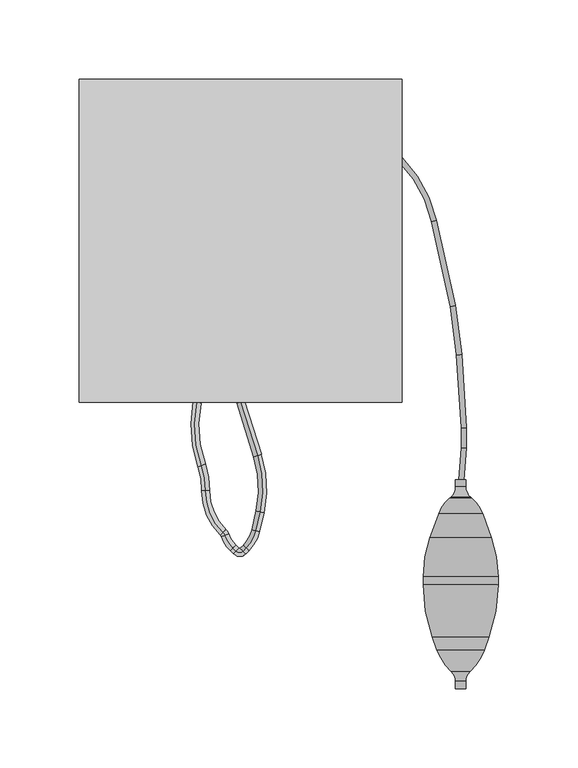
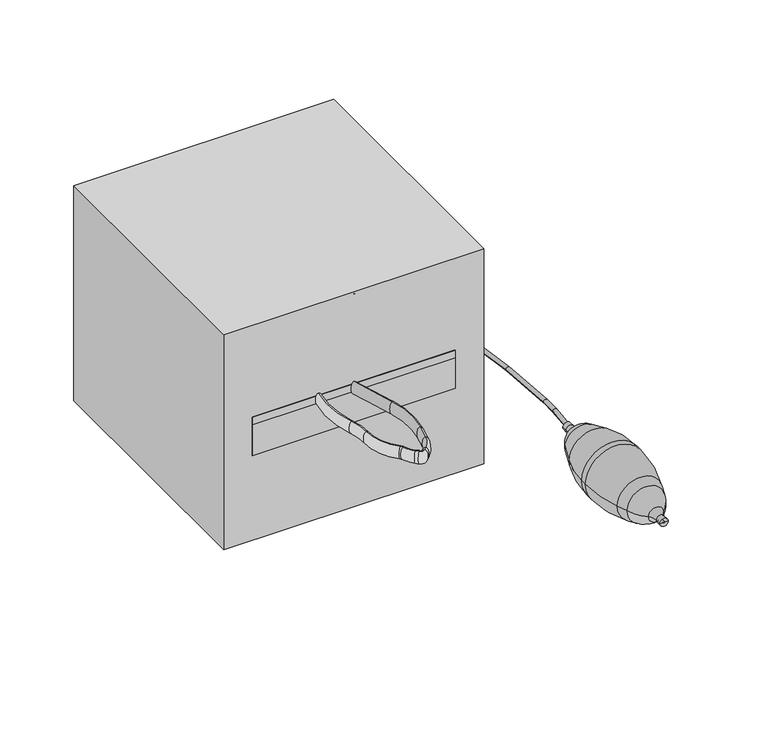
"""IFC4 building model written with IfcOpenShell, lengths in millimetres: proxy geometry, M4100 - Sphygmomanometer, Aneroid, Wall-Mounted : M4100 - Sphygmomanometer, Aneroid, Wall-Mounted."""

import ifcopenshell
import ifcopenshell.guid

model = None  # the IFC model being written
_history = None  # IfcOwnerHistory: only IFC2X3 demands one
_inside = {}  # id of a spatial element -> (the spatial element, [elements in it])
_under = {}  # id of a project, library or spatial element -> (it, [spatial elements below it])
_declared = {}  # id of a project -> (the project, [libraries it declares])
_typed = {}  # id of a type object -> (the type object, [elements of that type])
_made_of = {}  # id of a material, layer set ... -> (it, [elements and type objects made of it])


def new_model(schema):
    """Start an empty IFC model of exactly this schema.

    Asked for "IFC4X3", IfcOpenShell would pick the latest addendum, in which some entities
    have other attributes; the version numbers below select the first issue.
    IFC2X3 requires an IfcOwnerHistory on every rooted entity: one is made here for all.
    """
    global model, _history
    if schema == "IFC4X3":
        model = ifcopenshell.file(schema_version=(4, 3, 0, 0))
    else:
        model = ifcopenshell.file(schema=schema)
    _inside.clear()
    _under.clear()
    _declared.clear()
    _typed.clear()
    _made_of.clear()
    _history = None
    if model.schema == "IFC2X3":
        org = make("IfcOrganization", Name="unknown")
        user = make(
            "IfcPersonAndOrganization",
            ThePerson=make("IfcPerson", FamilyName="unknown"),
            TheOrganization=org,
        )
        app = make(
            "IfcApplication",
            ApplicationDeveloper=org,
            Version="unknown",
            ApplicationFullName="unknown",
            ApplicationIdentifier="unknown",
        )
        _history = make(
            "IfcOwnerHistory",
            OwningUser=user,
            OwningApplication=app,
            ChangeAction="ADDED",
            CreationDate=0,
        )
    return model


def make(cls, **values):
    """One entity of the class cls with the attributes given. An attribute that is None is left unset."""
    return model.create_entity(
        cls, **{name: value for name, value in values.items() if value is not None}
    )


def rooted(cls, **values):
    """An entity with a GlobalId (a new one), such as an element, a storey or a relation."""
    return make(cls, GlobalId=ifcopenshell.guid.new(), OwnerHistory=_history, **values)


def si_unit(unit_type, name, prefix=None):
    """IfcSIUnit, for example si_unit("LENGTHUNIT", "METRE", prefix="MILLI")."""
    return make("IfcSIUnit", UnitType=unit_type, Prefix=prefix, Name=name)


def assignment(units):
    """IfcUnitAssignment: the units of a project."""
    return None if units is None else make("IfcUnitAssignment", Units=units)


def point(xyz):
    """IfcCartesianPoint."""
    return None if xyz is None else make("IfcCartesianPoint", Coordinates=xyz)


def direction(xyz):
    """IfcDirection."""
    return None if xyz is None else make("IfcDirection", DirectionRatios=xyz)


def frame(location, z_axis=None, x_axis=None):
    """IfcAxis2Placement3D, a coordinate frame: its origin and axes. An axis left out is left unset."""
    return make(
        "IfcAxis2Placement3D",
        Location=point(location),
        Axis=direction(z_axis),
        RefDirection=direction(x_axis),
    )


def frame_2d(location, x_axis=None):
    """IfcAxis2Placement2D, a coordinate frame in the plane: its origin and x axis."""
    return make(
        "IfcAxis2Placement2D", Location=point(location), RefDirection=direction(x_axis)
    )


def origin():
    """The frame at (0, 0, 0) with its axes left unset."""
    return frame((0.0, 0.0, 0.0))


def origin_with_axes():
    """The frame at (0, 0, 0) with the z axis (0, 0, 1) and the x axis (1, 0, 0) written out."""
    return frame((0.0, 0.0, 0.0), z_axis=(0.0, 0.0, 1.0), x_axis=(1.0, 0.0, 0.0))


def place(relative_to, where):
    """IfcLocalPlacement: puts the frame where relative to a parent placement (None: the world)."""
    return make(
        "IfcLocalPlacement", PlacementRelTo=relative_to, RelativePlacement=where
    )


def context(
    kind, dimensions, precision=None, world=None, true_north=None, identifier=None
):
    """IfcGeometricRepresentationContext, for example the 3D "Model" context."""
    return make(
        "IfcGeometricRepresentationContext",
        ContextIdentifier=identifier,
        ContextType=kind,
        CoordinateSpaceDimension=dimensions,
        Precision=precision,
        WorldCoordinateSystem=world,
        TrueNorth=true_north,
    )


def project(units=None, contexts=None):
    """IfcProject with its units and contexts."""
    return rooted(
        "IfcProject",
        Name="project",
        RepresentationContexts=contexts,
        UnitsInContext=assignment(units),
    )


def spatial(cls, under=None, at=None, **own):
    """A site, building, storey or space (cls), placed at a placement, below another one or the project."""
    s = rooted(cls, ObjectPlacement=at, **own)
    if under is not None:
        _under.setdefault(under.id(), (under, []))[1].append(s)
    return s


def polyline(points):
    """IfcPolyline through the points."""
    return make("IfcPolyline", Points=[point(p) for p in points])


def circle_curve(where, radius):
    """IfcCircle in the frame where."""
    return make("IfcCircle", Position=where, Radius=radius)


def ellipse_curve(where, semi_axis1, semi_axis2):
    """IfcEllipse in the frame where."""
    return make(
        "IfcEllipse", Position=where, SemiAxis1=semi_axis1, SemiAxis2=semi_axis2
    )


def trimmed(basis, trim1, trim2, sense, master):
    """IfcTrimmedCurve: the piece of a basis curve between two trims."""
    return make(
        "IfcTrimmedCurve",
        BasisCurve=basis,
        Trim1=trim1,
        Trim2=trim2,
        SenseAgreement=sense,
        MasterRepresentation=master,
    )


def segment(curve, same_sense, transition):
    """IfcCompositeCurveSegment."""
    return make(
        "IfcCompositeCurveSegment",
        Transition=transition,
        SameSense=same_sense,
        ParentCurve=curve,
    )


def composite_curve(segments, self_intersect=None):
    """IfcCompositeCurve: segments joined end to end."""
    return make("IfcCompositeCurve", Segments=segments, SelfIntersect=self_intersect)


def outline(outer, holes=None, kind="AREA"):
    """IfcArbitraryClosedProfileDef: a profile drawn as a closed curve; with holes, ...WithVoids."""
    if holes is None:
        return make("IfcArbitraryClosedProfileDef", ProfileType=kind, OuterCurve=outer)
    return make(
        "IfcArbitraryProfileDefWithVoids",
        ProfileType=kind,
        OuterCurve=outer,
        InnerCurves=holes,
    )


def extrude(swept, where, along, depth):
    """IfcExtrudedAreaSolid: the profile swept, set in the frame where, extruded along a direction by depth."""
    return make(
        "IfcExtrudedAreaSolid",
        SweptArea=swept,
        Position=where,
        ExtrudedDirection=direction(along),
        Depth=depth,
    )


def shape(context_of_items, identifier, shape_type, items):
    """IfcShapeRepresentation: the items that make up one representation, for example the "Body"."""
    return make(
        "IfcShapeRepresentation",
        ContextOfItems=context_of_items,
        RepresentationIdentifier=identifier,
        RepresentationType=shape_type,
        Items=items,
    )


def source(mapping_origin, context_of_items, identifier, shape_type, items):
    """IfcRepresentationMap: a shape defined once, which mapped items show again and again."""
    return make(
        "IfcRepresentationMap",
        MappingOrigin=mapping_origin,
        MappedRepresentation=shape(context_of_items, identifier, shape_type, items),
    )


def transform(
    local_origin,
    x_axis=None,
    y_axis=None,
    z_axis=None,
    scale=None,
    scale2=None,
    scale3=None,
    uniform=True,
):
    """IfcCartesianTransformationOperator3D, or its non-uniform kind. x_axis, y_axis, z_axis: its Axis1, 2, 3."""
    if uniform:
        return make(
            "IfcCartesianTransformationOperator3D",
            Axis1=direction(x_axis),
            Axis2=direction(y_axis),
            LocalOrigin=point(local_origin),
            Scale=scale,
            Axis3=direction(z_axis),
        )
    return make(
        "IfcCartesianTransformationOperator3DnonUniform",
        Axis1=direction(x_axis),
        Axis2=direction(y_axis),
        LocalOrigin=point(local_origin),
        Scale=scale,
        Axis3=direction(z_axis),
        Scale2=scale2,
        Scale3=scale3,
    )


def mapped(mapping_source, mapping_target):
    """IfcMappedItem: shows the shape of a source again, moved by a transform."""
    return make(
        "IfcMappedItem", MappingSource=mapping_source, MappingTarget=mapping_target
    )


def made_of(thing, what):
    """Note that an element or type object is made of a material, layer set ...; save() writes the relation."""
    if what is not None:
        _made_of.setdefault(what.id(), (what, []))[1].append(thing)
    return thing


def element(
    cls,
    number,
    at=None,
    inside=None,
    cuts=None,
    type_object=None,
    material=None,
    context=None,
    identifier="Body",
    shape_type=None,
    held_by="IfcProductDefinitionShape",
    body=None,
    shapes=None,
    **own,
):
    """One element of the class cls, such as IfcWall. Its Tag is "e" and its number.

    at: its placement. inside: the storey or other place that contains it. cuts: it is an
    opening in that element (IfcRelVoidsElement). A single representation is given by context,
    identifier, shape_type and body (its items); several are given by shapes. held_by: the class
    of the entity that holds the representations. save() writes the other relations.
    """
    e = rooted(cls, Tag="e%d" % number, ObjectPlacement=at, **own)
    if body is not None:
        shapes = [shape(context, identifier, shape_type, body)]
    if shapes is not None:
        e.Representation = make(held_by, Representations=shapes)
    if inside is not None:
        _inside.setdefault(inside.id(), (inside, []))[1].append(e)
    if cuts is not None:
        rooted(
            "IfcRelVoidsElement", RelatingBuildingElement=cuts, RelatedOpeningElement=e
        )
    if type_object is not None:
        _typed.setdefault(type_object.id(), (type_object, []))[1].append(e)
    return made_of(e, material)


def aggregate(whole, parts):
    """IfcRelAggregates: a whole, such as a stair, and the parts it consists of."""
    return rooted("IfcRelAggregates", RelatingObject=whole, RelatedObjects=parts)


def save(model, path):
    """Write the relations noted so far, then the file.

    IfcRelAggregates (storeys below a building ...), IfcRelContainedInSpatialStructure (elements
    in a storey), IfcRelDefinesByType, IfcRelAssociatesMaterial and IfcRelDeclares: one each for
    every whole, place, type object, material and project.
    """
    for whole, parts in _under.values():
        aggregate(whole, parts)
    for where, things in _inside.values():
        rooted(
            "IfcRelContainedInSpatialStructure",
            RelatedElements=things,
            RelatingStructure=where,
        )
    for kind, things in _typed.values():
        rooted("IfcRelDefinesByType", RelatedObjects=things, RelatingType=kind)
    for what, things in _made_of.values():
        rooted("IfcRelAssociatesMaterial", RelatedObjects=things, RelatingMaterial=what)
    for by, libraries in _declared.values():
        rooted("IfcRelDeclares", RelatingContext=by, RelatedDefinitions=libraries)
    model.write(path)


def plane_surface(at):
    """IfcPlane: the flat surface through the origin of the frame at, square to its z axis."""
    return make("IfcPlane", Position=at)


def cylinder_surface(at, radius):
    """IfcCylindricalSurface: all points at the distance radius from the z axis of the frame at."""
    return make("IfcCylindricalSurface", Position=at, Radius=radius)


def revolved_surface(curve, axis_point, axis_direction):
    """IfcSurfaceOfRevolution: the curve turned about the line through axis_point along axis_direction."""
    return make(
        "IfcSurfaceOfRevolution",
        SweptCurve=make("IfcArbitraryOpenProfileDef", ProfileType="CURVE", Curve=curve),
        AxisPosition=make("IfcAxis1Placement", Location=point(axis_point), Axis=direction(axis_direction)),
    )


def extruded_surface(curve, direction_of_extrusion, depth):
    """IfcSurfaceOfLinearExtrusion: the curve pushed along a direction by depth."""
    return make(
        "IfcSurfaceOfLinearExtrusion",
        SweptCurve=make("IfcArbitraryOpenProfileDef", ProfileType="CURVE", Curve=curve),
        ExtrudedDirection=direction(direction_of_extrusion),
        Depth=depth,
    )


def advanced_brep(points, edges, surfaces, faces):
    """IfcAdvancedBrep: a solid bounded by faces that lie on surfaces and meet in shared edges.

    An edge is (start, end): straight between two places in points (the first is 0);
    or (start, end, curve); or (start, end, curve, False) where it runs against its curve.
    A face is (place in surfaces, loops), or (place, loops, False) where it looks against
    its surface's normal. A loop lists edges by number (the first is 1), with a minus sign
    where the edge is run from its end to its start. The first loop is the outer one.
    """
    corners = [point(p) for p in points]
    vertices = [make("IfcVertexPoint", VertexGeometry=c) for c in corners]
    made = []
    for start, end, *more in edges:
        made.append(
            make(
                "IfcEdgeCurve",
                EdgeStart=vertices[start],
                EdgeEnd=vertices[end],
                EdgeGeometry=more[0] if more else make("IfcPolyline", Points=[corners[start], corners[end]]),
                SameSense=more[1] if len(more) > 1 else True,
            )
        )
    hull = []
    for where, loops, *sense in faces:
        bounds = []
        for j, loop in enumerate(loops):
            ring = [make("IfcOrientedEdge", EdgeElement=made[abs(k) - 1], Orientation=k > 0) for k in loop]
            bounds.append(
                make(
                    "IfcFaceOuterBound" if j == 0 else "IfcFaceBound",
                    Bound=make("IfcEdgeLoop", EdgeList=ring),
                    Orientation=True,
                )
            )
        hull.append(make("IfcAdvancedFace", Bounds=bounds, FaceSurface=surfaces[where], SameSense=sense[0] if sense else True))
    return make("IfcAdvancedBrep", Outer=make("IfcClosedShell", CfsFaces=hull))


def specialty_equipment_8f949246(model_context):
    return source(origin(), model_context, "Body", "SolidModel", [
        advanced_brep(
        [(0.0, 0.0, 93.3890108), (0.0, 0.0, 103.4609892), (10.60129, -33.4899695, 93.3890108), (10.60129, -33.4899695, 103.4609892), (12.1452256, -68.8519095, 103.4609892), (12.1452256, -68.8519095, 93.3890108), (9.4902706, -80.7634297, 93.3890108), (9.4902706, -80.7634297, 103.4609892), (3.5257448, -91.6206606, 103.4609892), (3.5257448, -91.6206606, 93.3890108), (1.489236, -93.6571694, 93.3890108), (1.489236, -93.6571694, 103.4609892), (-2.7411458, -93.6571694, 103.4609892), (-2.7411458, -93.6571694, 93.3890108), (-4.6658712, -91.732444, 93.3890108), (-4.6658712, -91.732444, 103.4609892), (-9.7582734, -83.8141156, 103.4609892), (-9.7582734, -83.8141156, 93.3890108), (-10.9708227, -81.9675873, 103.4609892), (-10.9708227, -81.9675873, 93.3890108), (-21.9594666, -55.7504476, 103.4609892), (-21.9594666, -55.7504476, 93.3890108), (-24.5939327, -39.9510684, 103.4609892), (-24.5939327, -39.9510684, 93.3890108), (-27.3580457, -0.1117834, 93.3890108), (-27.3580457, -0.1117834, 103.4609892)],
        [
            (0, 1, ellipse_curve(frame((0.0, 0.0, 98.425), z_axis=(-0.30179165133573443, 0.9533739031377199, 0.0), x_axis=(0.0, 0.0, 1.0)), 5.0359892, 2.5179946)),
            (1, 0, ellipse_curve(frame((0.0, 0.0, 98.425), z_axis=(-0.30179165133573443, 0.9533739031377199, 0.0), x_axis=(0.0, 0.0, 1.0)), 5.0359892, 2.5179946)),
            (0, 2),
            (2, 3, ellipse_curve(frame((10.60129, -33.4899695, 98.425), z_axis=(-0.3017916513357344, 0.9533739031377201, 0.0), x_axis=(0.0, 0.0, 1.0)), 5.0359892, 2.5179946)),
            (3, 1),
            (3, 2, ellipse_curve(frame((10.60129, -33.4899695, 98.425), z_axis=(-0.3017916513357344, 0.9533739031377201, 0.0), x_axis=(0.0, 0.0, 1.0)), 5.0359892, 2.5179946)),
            (4, 3, circle_curve(frame((-54.3137244, -54.0388951, 103.4609892), z_axis=(0.0, 0.0, 1.0), x_axis=(0.9533739031377199, 0.3017916513357344, 0.0)), 68.0897748)),
            (2, 5, circle_curve(frame((-54.3137244, -54.0388951, 93.3890108), z_axis=(0.0, 0.0, -1.0), x_axis=(0.9533739031377199, 0.3017916513357344, 0.0)), 68.0897748)),
            (5, 4, ellipse_curve(frame((12.1452256, -68.8519095, 98.425), z_axis=(0.21755123234481044, 0.9760489031320381, 0.0), x_axis=(0.0, 0.0, 1.0)), 5.0359892, 2.5179946)),
            (4, 5, ellipse_curve(frame((12.1452256, -68.8519095, 98.425), z_axis=(0.21755123234481044, 0.9760489031320381, 0.0), x_axis=(0.0, 0.0, 1.0)), 5.0359892, 2.5179946)),
            (5, 6),
            (6, 7, ellipse_curve(frame((9.4902706, -80.7634297, 98.425), z_axis=(0.21755123234481058, 0.9760489031320381, 0.0), x_axis=(0.0, 0.0, 1.0)), 5.0359892, 2.5179946)),
            (7, 4),
            (7, 6, ellipse_curve(frame((9.4902706, -80.7634297, 98.425), z_axis=(0.21755123234481058, 0.9760489031320381, 0.0), x_axis=(0.0, 0.0, 1.0)), 5.0359892, 2.5179946)),
            (8, 7, circle_curve(frame((-12.1562786, -75.9386371, 103.4609892), z_axis=(0.0, 0.0, 1.0), x_axis=(0.9760489031320378, -0.21755123234481052, 0.0)), 22.1777302)),
            (6, 9, circle_curve(frame((-12.1562786, -75.9386371, 93.3890108), z_axis=(0.0, 0.0, -1.0), x_axis=(0.9760489031320378, -0.21755123234481052, 0.0)), 22.1777302)),
            (9, 8, ellipse_curve(frame((3.5257448, -91.6206606, 98.425), z_axis=(0.7071067811865471, 0.7071067811865479, 0.0), x_axis=(0.0, 0.0, 1.0)), 5.0359892, 2.5179946)),
            (8, 9, ellipse_curve(frame((3.5257448, -91.6206606, 98.425), z_axis=(0.7071067811865478, 0.7071067811865472, 0.0), x_axis=(0.0, 0.0, 1.0)), 5.0359892, 2.5179946)),
            (9, 10),
            (10, 11, ellipse_curve(frame((1.489236, -93.6571694, 98.425), z_axis=(0.7071067811865424, 0.7071067811865528, 0.0), x_axis=(0.0, 0.0, 1.0)), 5.0359892, 2.5179946)),
            (11, 8),
            (11, 10, ellipse_curve(frame((1.489236, -93.6571694, 98.425), z_axis=(0.7071067811865424, 0.7071067811865528, 0.0), x_axis=(0.0, 0.0, 1.0)), 5.0359892, 2.5179946)),
            (12, 11, circle_curve(frame((-0.6259549, -91.5419785, 103.4609892), z_axis=(0.0, 0.0, 1.0), x_axis=(0.7071067811865528, -0.7071067811865424, 0.0)), 2.9913317)),
            (10, 13, circle_curve(frame((-0.6259549, -91.5419785, 93.3890108), z_axis=(0.0, 0.0, -1.0), x_axis=(0.7071067811865528, -0.7071067811865424, 0.0)), 2.9913317)),
            (13, 12, ellipse_curve(frame((-2.7411458, -93.6571694, 98.425), z_axis=(0.7071067811865399, -0.7071067811865552, 0.0), x_axis=(0.0, 0.0, 1.0)), 5.0359892, 2.5179946)),
            (12, 13, ellipse_curve(frame((-2.7411458, -93.6571694, 98.425), z_axis=(0.7071067811865431, -0.707106781186552, 0.0), x_axis=(0.0, 0.0, 1.0)), 5.0359892, 2.5179946)),
            (13, 14),
            (14, 15, ellipse_curve(frame((-4.6658712, -91.732444, 98.425), z_axis=(0.7071067811865434, -0.7071067811865517, 0.0), x_axis=(0.0, 0.0, 1.0)), 5.0359892, 2.5179946)),
            (15, 12),
            (15, 14, ellipse_curve(frame((-4.6658712, -91.732444, 98.425), z_axis=(0.7071067811865434, -0.7071067811865517, 0.0), x_axis=(0.0, 0.0, 1.0)), 5.0359892, 2.5179946)),
            (16, 15, circle_curve(frame((11.0161522, -76.0504205, 103.4609892), z_axis=(0.0, 0.0, 1.0), x_axis=(-0.7071067811865517, -0.7071067811865434, 0.0)), 22.1777302)),
            (14, 17, circle_curve(frame((11.0161522, -76.0504205, 93.3890108), z_axis=(0.0, 0.0, -1.0), x_axis=(-0.7071067811865517, -0.7071067811865434, 0.0)), 22.1777302)),
            (17, 16, ellipse_curve(frame((-9.7582734, -83.8141156, 98.425), z_axis=(0.3500671620040357, -0.9367246031179284, 0.0), x_axis=(0.0, 0.0, 1.0)), 5.0359892, 2.5179946)),
            (16, 17, ellipse_curve(frame((-9.7582734, -83.8141156, 98.425), z_axis=(0.35006716200403576, -0.9367246031179283, 0.0), x_axis=(0.0, 0.0, 1.0)), 5.0359892, 2.5179946)),
            (18, 16, circle_curve(frame((-14.4282922, -85.5593673, 103.4609892), z_axis=(0.0, 0.0, -1.0), x_axis=(0.9367246031179312, 0.3500671620040279, 0.0)), 4.9854768)),
            (17, 19, circle_curve(frame((-14.4282922, -85.5593673, 93.3890108), z_axis=(0.0, 0.0, 1.0), x_axis=(0.9367246031179312, 0.3500671620040279, 0.0)), 4.9854768)),
            (19, 18, ellipse_curve(frame((-10.9708227, -81.9675873, 98.425), z_axis=(0.720448655639569, -0.6935082801143313, 0.0), x_axis=(0.0, 0.0, 1.0)), 5.0359892, 2.5179946)),
            (18, 19, ellipse_curve(frame((-10.9708227, -81.9675873, 98.425), z_axis=(0.7204486556395685, -0.6935082801143317, 0.0), x_axis=(0.0, 0.0, 1.0)), 5.0359892, 2.5179946)),
            (20, 18, circle_curve(frame((13.8981281, -56.1325645, 103.4609892), z_axis=(0.0, 0.0, 1.0), x_axis=(-0.6935082801143324, -0.7204486556395678, 0.0)), 35.8596307)),
            (19, 21, circle_curve(frame((13.8981281, -56.1325645, 93.3890108), z_axis=(0.0, 0.0, -1.0), x_axis=(-0.6935082801143324, -0.7204486556395678, 0.0)), 35.8596307)),
            (21, 20, ellipse_curve(frame((-21.9594666, -55.7504476, 98.425), z_axis=(-0.010655908230738531, -0.9999432241981432, 0.0), x_axis=(0.0, 0.0, 1.0)), 5.0359892, 2.5179946)),
            (20, 21, ellipse_curve(frame((-21.9594666, -55.7504476, 98.425), z_axis=(-0.010655908230738531, -0.9999432241981432, 0.0), x_axis=(0.0, 0.0, 1.0)), 5.0359892, 2.5179946)),
            (22, 20, circle_curve(frame((-67.7275968, -55.2627189, 103.4609892), z_axis=(0.0, 0.0, -1.0), x_axis=(0.9999432241981431, -0.010655908230754234, 0.0)), 45.7707289)),
            (21, 23, circle_curve(frame((-67.7275968, -55.2627189, 93.3890108), z_axis=(0.0, 0.0, 1.0), x_axis=(0.9999432241981431, -0.010655908230754234, 0.0)), 45.7707289)),
            (23, 22, ellipse_curve(frame((-24.5939327, -39.9510684, 98.425), z_axis=(0.33452931398523167, -0.9423853447950952, 0.0), x_axis=(0.0, 0.0, 1.0)), 5.0359892, 2.5179946)),
            (22, 23, ellipse_curve(frame((-24.5939327, -39.9510684, 98.425), z_axis=(0.33452931398523156, -0.9423853447950952, 0.0), x_axis=(0.0, 0.0, 1.0)), 5.0359892, 2.5179946)),
            (24, 25, ellipse_curve(frame((-27.3580457, -0.1117834, 98.425), z_axis=(0.2011821163330489, 0.9795538556239548, 0.0), x_axis=(0.0, 0.0, 1.0)), 5.0359892, 2.5179946)),
            (25, 24, ellipse_curve(frame((-27.3580457, -0.1117834, 98.425), z_axis=(0.2011821163330489, 0.9795538556239548, 0.0), x_axis=(0.0, 0.0, 1.0)), 5.0359892, 2.5179946)),
            (25, 22, circle_curve(frame((45.4884963, -15.0731063, 103.4609892), z_axis=(0.0, 0.0, 1.0), x_axis=(-0.9423853447950952, -0.33452931398523145, 0.0)), 74.3670617)),
            (23, 24, circle_curve(frame((45.4884963, -15.0731063, 93.3890108), z_axis=(0.0, 0.0, -1.0), x_axis=(-0.9423853447950952, -0.33452931398523145, 0.0)), 74.3670617)),
        ],
        [
            plane_surface(frame((0.0, 0.0, 98.425), z_axis=(-0.30179165133573443, 0.9533739031377199, 0.0), x_axis=(0.0, 0.0, 1.0))),
            extruded_surface(trimmed(ellipse_curve(frame((10.60129, -33.4899695, 98.425), z_axis=(-0.30179165133573443, 0.9533739031377199, 0.0), x_axis=(0.0, 0.0, 1.0)), 5.0359892, 2.5179946), [point((10.60129, -33.4899695, 93.3890108))], [point((10.60129, -33.4899695, 103.4609892))], True, "CARTESIAN"), (-10.60129, 33.4899695, 0.0), 35.1278437535672),
            extruded_surface(trimmed(ellipse_curve(frame((10.60129, -33.4899695, 98.425), z_axis=(-0.30179165133573443, 0.9533739031377199, 0.0), x_axis=(0.0, 0.0, 1.0)), 5.0359892, 2.5179946), [point((10.60129, -33.4899695, 103.4609892))], [point((10.60129, -33.4899695, 93.3890108))], True, "CARTESIAN"), (-10.60129, 33.4899695, 0.0), 35.1278437535672),
            revolved_surface(trimmed(ellipse_curve(frame((10.60129, -33.4899695, 98.425), z_axis=(-0.3017916513357343, 0.9533739031377199, 0.0), x_axis=(0.0, 0.0, 1.0)), 5.0359892, 2.5179946), [point((10.60129, -33.4899695, 93.3890108))], [point((10.60129, -33.4899695, 103.4609892))], True, "CARTESIAN"), (-54.3137244, -54.0388951, 98.425), (0.0, 0.0, -1.0)),
            revolved_surface(trimmed(ellipse_curve(frame((10.60129, -33.4899695, 98.425), z_axis=(-0.3017916513357343, 0.9533739031377199, 0.0), x_axis=(0.0, 0.0, 1.0)), 5.0359892, 2.5179946), [point((10.60129, -33.4899695, 103.4609892))], [point((10.60129, -33.4899695, 93.3890108))], True, "CARTESIAN"), (-54.3137244, -54.0388951, 98.425), (0.0, 0.0, -1.0)),
            extruded_surface(trimmed(ellipse_curve(frame((9.4902706, -80.7634297, 98.425), z_axis=(0.2175512323448103, 0.976048903132038, 0.0), x_axis=(0.0, 0.0, 1.0)), 5.0359892, 2.5179946), [point((9.4902706, -80.7634297, 93.3890108))], [point((9.4902706, -80.7634297, 103.4609892))], True, "CARTESIAN"), (2.6549549999999993, 11.911520199999998, 0.0), 12.203814957915126),
            extruded_surface(trimmed(ellipse_curve(frame((9.4902706, -80.7634297, 98.425), z_axis=(0.2175512323448103, 0.976048903132038, 0.0), x_axis=(0.0, 0.0, 1.0)), 5.0359892, 2.5179946), [point((9.4902706, -80.7634297, 103.4609892))], [point((9.4902706, -80.7634297, 93.3890108))], True, "CARTESIAN"), (2.6549549999999993, 11.911520199999998, 0.0), 12.203814957915126),
            revolved_surface(trimmed(ellipse_curve(frame((9.4902706, -80.7634297, 98.425), z_axis=(0.21755123234481052, 0.9760489031320378, 0.0), x_axis=(0.0, 0.0, 1.0)), 5.0359892, 2.5179946), [point((9.4902706, -80.7634297, 93.3890108))], [point((9.4902706, -80.7634297, 103.4609892))], True, "CARTESIAN"), (-12.1562786, -75.9386371, 98.425), (0.0, 0.0, -1.0)),
            revolved_surface(trimmed(ellipse_curve(frame((9.4902706, -80.7634297, 98.425), z_axis=(0.21755123234481052, 0.9760489031320378, 0.0), x_axis=(0.0, 0.0, 1.0)), 5.0359892, 2.5179946), [point((9.4902706, -80.7634297, 103.4609892))], [point((9.4902706, -80.7634297, 93.3890108))], True, "CARTESIAN"), (-12.1562786, -75.9386371, 98.425), (0.0, 0.0, -1.0)),
            extruded_surface(trimmed(ellipse_curve(frame((1.489236, -93.6571694, 98.425), z_axis=(0.707106781186548, 0.707106781186547, 0.0), x_axis=(0.0, 0.0, 1.0)), 5.0359892, 2.5179946), [point((1.489236, -93.6571694, 93.3890108))], [point((1.489236, -93.6571694, 103.4609892))], True, "CARTESIAN"), (2.0365088, 2.036508800000007, 0.0), 2.8800583648521623),
            extruded_surface(trimmed(ellipse_curve(frame((1.489236, -93.6571694, 98.425), z_axis=(0.707106781186548, 0.707106781186547, 0.0), x_axis=(0.0, 0.0, 1.0)), 5.0359892, 2.5179946), [point((1.489236, -93.6571694, 103.4609892))], [point((1.489236, -93.6571694, 93.3890108))], True, "CARTESIAN"), (2.0365088, 2.036508800000007, 0.0), 2.8800583648521623),
            revolved_surface(trimmed(ellipse_curve(frame((1.489236, -93.6571694, 98.425), z_axis=(0.7071067811865424, 0.7071067811865528, 0.0), x_axis=(0.0, 0.0, 1.0)), 5.0359892, 2.5179946), [point((1.489236, -93.6571694, 93.3890108))], [point((1.489236, -93.6571694, 103.4609892))], True, "CARTESIAN"), (-0.6259549, -91.5419785, 98.425), (0.0, 0.0, -1.0)),
            revolved_surface(trimmed(ellipse_curve(frame((1.489236, -93.6571694, 98.425), z_axis=(0.7071067811865424, 0.7071067811865528, 0.0), x_axis=(0.0, 0.0, 1.0)), 5.0359892, 2.5179946), [point((1.489236, -93.6571694, 103.4609892))], [point((1.489236, -93.6571694, 93.3890108))], True, "CARTESIAN"), (-0.6259549, -91.5419785, 98.425), (0.0, 0.0, -1.0)),
            extruded_surface(trimmed(ellipse_curve(frame((-4.6658712, -91.732444, 98.425), z_axis=(0.707106781186542, -0.7071067811865531, 0.0), x_axis=(0.0, 0.0, 1.0)), 5.0359892, 2.5179946), [point((-4.6658712, -91.732444, 93.3890108))], [point((-4.6658712, -91.732444, 103.4609892))], True, "CARTESIAN"), (1.9247253999999998, -1.9247253999999998, 0.0), 2.72197276452398),
            extruded_surface(trimmed(ellipse_curve(frame((-4.6658712, -91.732444, 98.425), z_axis=(0.707106781186542, -0.7071067811865531, 0.0), x_axis=(0.0, 0.0, 1.0)), 5.0359892, 2.5179946), [point((-4.6658712, -91.732444, 103.4609892))], [point((-4.6658712, -91.732444, 93.3890108))], True, "CARTESIAN"), (1.9247253999999998, -1.9247253999999998, 0.0), 2.72197276452398),
            revolved_surface(trimmed(ellipse_curve(frame((-4.6658712, -91.732444, 98.425), z_axis=(0.7071067811865434, -0.7071067811865517, 0.0), x_axis=(0.0, 0.0, 1.0)), 5.0359892, 2.5179946), [point((-4.6658712, -91.732444, 93.3890108))], [point((-4.6658712, -91.732444, 103.4609892))], True, "CARTESIAN"), (11.0161522, -76.0504205, 98.425), (0.0, 0.0, -1.0)),
            revolved_surface(trimmed(ellipse_curve(frame((-4.6658712, -91.732444, 98.425), z_axis=(0.7071067811865434, -0.7071067811865517, 0.0), x_axis=(0.0, 0.0, 1.0)), 5.0359892, 2.5179946), [point((-4.6658712, -91.732444, 103.4609892))], [point((-4.6658712, -91.732444, 93.3890108))], True, "CARTESIAN"), (11.0161522, -76.0504205, 98.425), (0.0, 0.0, -1.0)),
            revolved_surface(trimmed(ellipse_curve(frame((-9.7582734, -83.8141156, 98.425), z_axis=(0.350067162004028, -0.9367246031179312, 0.0), x_axis=(0.0, 0.0, 1.0)), 5.0359892, 2.5179946), [point((-9.7582734, -83.8141156, 93.3890108))], [point((-9.7582734, -83.8141156, 103.4609892))], True, "CARTESIAN"), (-14.4282922, -85.5593673, 98.425), (0.0, 0.0, 1.0)),
            revolved_surface(trimmed(ellipse_curve(frame((-9.7582734, -83.8141156, 98.425), z_axis=(0.350067162004028, -0.9367246031179312, 0.0), x_axis=(0.0, 0.0, 1.0)), 5.0359892, 2.5179946), [point((-9.7582734, -83.8141156, 103.4609892))], [point((-9.7582734, -83.8141156, 93.3890108))], True, "CARTESIAN"), (-14.4282922, -85.5593673, 98.425), (0.0, 0.0, 1.0)),
            revolved_surface(trimmed(ellipse_curve(frame((-10.9708227, -81.9675873, 98.425), z_axis=(0.7204486556395681, -0.6935082801143322, 0.0), x_axis=(0.0, 0.0, 1.0)), 5.0359892, 2.5179946), [point((-10.9708227, -81.9675873, 93.3890108))], [point((-10.9708227, -81.9675873, 103.4609892))], True, "CARTESIAN"), (13.8981281, -56.1325645, 98.425), (0.0, 0.0, -1.0)),
            revolved_surface(trimmed(ellipse_curve(frame((-10.9708227, -81.9675873, 98.425), z_axis=(0.7204486556395681, -0.6935082801143322, 0.0), x_axis=(0.0, 0.0, 1.0)), 5.0359892, 2.5179946), [point((-10.9708227, -81.9675873, 103.4609892))], [point((-10.9708227, -81.9675873, 93.3890108))], True, "CARTESIAN"), (13.8981281, -56.1325645, 98.425), (0.0, 0.0, -1.0)),
            revolved_surface(trimmed(ellipse_curve(frame((-21.9594666, -55.7504476, 98.425), z_axis=(-0.010655908230753961, -0.9999432241981431, 0.0), x_axis=(0.0, 0.0, 1.0)), 5.0359892, 2.5179946), [point((-21.9594666, -55.7504476, 93.3890108))], [point((-21.9594666, -55.7504476, 103.4609892))], True, "CARTESIAN"), (-67.7275968, -55.2627189, 98.425), (0.0, 0.0, 1.0)),
            revolved_surface(trimmed(ellipse_curve(frame((-21.9594666, -55.7504476, 98.425), z_axis=(-0.010655908230753961, -0.9999432241981431, 0.0), x_axis=(0.0, 0.0, 1.0)), 5.0359892, 2.5179946), [point((-21.9594666, -55.7504476, 103.4609892))], [point((-21.9594666, -55.7504476, 93.3890108))], True, "CARTESIAN"), (-67.7275968, -55.2627189, 98.425), (0.0, 0.0, 1.0)),
            plane_surface(frame((-27.3580457, -0.1117834, 98.425), z_axis=(0.201182116333049, 0.9795538556239548, 0.0), x_axis=(0.0, 0.0, 1.0))),
            revolved_surface(trimmed(ellipse_curve(frame((-24.5939327, -39.9510684, 98.425), z_axis=(0.3345293139852318, -0.9423853447950951, 0.0), x_axis=(0.0, 0.0, 1.0)), 5.0359892, 2.5179946), [point((-24.5939327, -39.9510684, 93.3890108))], [point((-24.5939327, -39.9510684, 103.4609892))], True, "CARTESIAN"), (45.4884963, -15.0731063, 98.425), (0.0, 0.0, -1.0)),
            revolved_surface(trimmed(ellipse_curve(frame((-24.5939327, -39.9510684, 98.425), z_axis=(0.3345293139852318, -0.9423853447950951, 0.0), x_axis=(0.0, 0.0, 1.0)), 5.0359892, 2.5179946), [point((-24.5939327, -39.9510684, 103.4609892))], [point((-24.5939327, -39.9510684, 93.3890108))], True, "CARTESIAN"), (45.4884963, -15.0731063, 98.425), (0.0, 0.0, -1.0)),
        ],
        [
            (0, [[1, 2]]),
            (1, [[-1, 3, 4, 5]]),
            (2, [[-2, -5, 6, -3]]),
            (3, [[7, -4, 8, 9]]),
            (4, [[-8, -6, -7, 10]]),
            (5, [[-9, 11, 12, 13]]),
            (6, [[-10, -13, 14, -11]]),
            (7, [[15, -12, 16, 17]]),
            (8, [[-16, -14, -15, 18]]),
            (9, [[-17, 19, 20, 21]]),
            (10, [[-18, -21, 22, -19]]),
            (11, [[23, -20, 24, 25]]),
            (12, [[-24, -22, -23, 26]]),
            (13, [[-25, 27, 28, 29]]),
            (14, [[-26, -29, 30, -27]]),
            (15, [[31, -28, 32, 33]]),
            (16, [[-32, -30, -31, 34]]),
            (17, [[35, -33, 36, 37]]),
            (18, [[-36, -34, -35, 38]]),
            (19, [[39, -37, 40, 41]]),
            (20, [[-40, -38, -39, 42]]),
            (21, [[43, -41, 44, 45]]),
            (22, [[-44, -42, -43, 46]]),
            (23, [[47, 48]]),
            (24, [[49, -45, 50, -48]]),
            (25, [[-50, -46, -49, -47]]),
        ],
    ),
        advanced_brep(
        [(138.1282079, -48.8005767, 47.6946196), (139.110677, -48.8005767, 47.6946196), (141.8571136, -48.8005767, 47.6946196), (135.3817713, -48.8005767, 47.6946196), (138.1282079, -180.1855223, 47.6946196), (139.110677, -180.1855223, 47.6946196), (135.3817713, -180.1855223, 47.6946196), (141.8571136, -180.1855223, 47.6946196), (135.3817713, -175.5632852, 47.6946196), (141.8571136, -175.5632852, 47.6946196), (132.7169258, -169.4696535, 47.6946196), (144.5219592, -169.4696535, 47.6946196), (123.7575473, -155.9951928, 47.6946196), (153.4813376, -155.9951928, 47.6946196), (120.8482177, -148.0018755, 47.6946196), (156.3906672, -148.0018755, 47.6946196), (114.9866942, -114.7595239, 47.6946196), (162.2521907, -114.7595239, 47.6946196), (114.9866942, -109.7483973, 47.6946196), (162.2521907, -109.7483973, 47.6946196), (119.3165907, -85.1923341, 47.6946196), (157.9222942, -85.1923341, 47.6946196), (124.8056359, -70.1113063, 47.6946196), (152.433249, -70.1113063, 47.6946196), (131.6106524, -60.3927356, 47.6946196), (145.6282325, -60.3927356, 47.6946196), (132.2844617, -59.8273424, 47.6946196), (144.9544232, -59.8273424, 47.6946196), (135.3817713, -53.1851407, 47.6946196), (141.8571136, -53.1851407, 47.6946196)],
        [
            (0, 1, circle_curve(frame((138.6194425, -48.8005767, 47.6946196), z_axis=(0.0, -1.0, 0.0), x_axis=(1.0, 0.0, 0.0)), 0.4912345)),
            (1, 2),
            (2, 3, circle_curve(frame((138.6194425, -48.8005767, 47.6946196), z_axis=(0.0, 1.0, 0.0), x_axis=(1.0, 0.0, 0.0)), 3.2376712)),
            (3, 0),
            (1, 0, circle_curve(frame((138.6194425, -48.8005767, 47.6946196), z_axis=(0.0, -1.0, 0.0), x_axis=(1.0, 0.0, 0.0)), 0.4912345)),
            (3, 2, circle_curve(frame((138.6194425, -48.8005767, 47.6946196), z_axis=(0.0, 1.0, 0.0), x_axis=(1.0, 0.0, 0.0)), 3.2376712)),
            (4, 5, circle_curve(frame((138.6194425, -180.1855223, 47.6946196), z_axis=(0.0, -1.0, 0.0), x_axis=(1.0, 0.0, 0.0)), 0.4912345)),
            (5, 1),
            (0, 4),
            (5, 4, circle_curve(frame((138.6194425, -180.1855223, 47.6946196), z_axis=(0.0, -1.0, 0.0), x_axis=(1.0, 0.0, 0.0)), 0.4912345)),
            (6, 7, circle_curve(frame((138.6194425, -180.1855223, 47.6946196), z_axis=(0.0, -1.0, 0.0), x_axis=(1.0, 0.0, 0.0)), 3.2376712)),
            (7, 5),
            (4, 6),
            (7, 6, circle_curve(frame((138.6194425, -180.1855223, 47.6946196), z_axis=(0.0, -1.0, 0.0), x_axis=(1.0, 0.0, 0.0)), 3.2376712)),
            (8, 9, circle_curve(frame((138.6194425, -175.5632852, 47.6946196), z_axis=(0.0, -1.0, 0.0), x_axis=(1.0, 0.0, 0.0)), 3.2376712)),
            (9, 7),
            (6, 8),
            (9, 8, circle_curve(frame((138.6194425, -175.5632852, 47.6946196), z_axis=(0.0, -1.0, 0.0), x_axis=(1.0, 0.0, 0.0)), 3.2376712)),
            (10, 11, circle_curve(frame((138.6194425, -169.4696535, 47.6946196), z_axis=(0.0, -1.0, 0.0), x_axis=(1.0, 0.0, 0.0)), 5.9025167)),
            (11, 9, circle_curve(frame((150.1566096, -175.5632852, 47.6946196), z_axis=(0.0, 0.0, 1.0), x_axis=(1.0, 0.0, 0.0)), 8.299496)),
            (8, 10, circle_curve(frame((127.0822753, -175.5632852, 47.6946196), z_axis=(0.0, 0.0, 1.0), x_axis=(-1.0, 0.0, 0.0)), 8.299496)),
            (11, 10, circle_curve(frame((138.6194425, -169.4696535, 47.6946196), z_axis=(0.0, -1.0, 0.0), x_axis=(1.0, 0.0, 0.0)), 5.9025167)),
            (12, 13, circle_curve(frame((138.6194425, -155.9951928, 47.6946196), z_axis=(0.0, -1.0, 0.0), x_axis=(1.0, 0.0, 0.0)), 14.8618952)),
            (13, 11, circle_curve(frame((121.1969167, -144.2446246, 47.6946196), z_axis=(0.0, 0.0, -1.0), x_axis=(1.0, 0.0, 0.0)), 34.3563632)),
            (10, 12, circle_curve(frame((156.0419683, -144.2446246, 47.6946196), z_axis=(0.0, 0.0, -1.0), x_axis=(-1.0, 0.0, 0.0)), 34.3563632)),
            (13, 12, circle_curve(frame((138.6194425, -155.9951928, 47.6946196), z_axis=(0.0, -1.0, 0.0), x_axis=(1.0, 0.0, 0.0)), 14.8618952)),
            (14, 15, circle_curve(frame((138.6194425, -148.0018755, 47.6946196), z_axis=(0.0, -1.0, 0.0), x_axis=(1.0, 0.0, 0.0)), 17.7712248)),
            (15, 13),
            (12, 14),
            (15, 14, circle_curve(frame((138.6194425, -148.0018755, 47.6946196), z_axis=(0.0, -1.0, 0.0), x_axis=(1.0, 0.0, 0.0)), 17.7712248)),
            (16, 17, circle_curve(frame((138.6194425, -114.7595239, 47.6946196), z_axis=(0.0, -1.0, 0.0), x_axis=(1.0, 0.0, 0.0)), 23.6327482)),
            (17, 15, circle_curve(frame((65.058057, -114.7595239, 47.6946196), z_axis=(0.0, 0.0, -1.0), x_axis=(1.0, 0.0, 0.0)), 97.1941337)),
            (14, 16, circle_curve(frame((212.1808279, -114.7595239, 47.6946196), z_axis=(0.0, 0.0, -1.0), x_axis=(-1.0, 0.0, 0.0)), 97.1941337)),
            (17, 16, circle_curve(frame((138.6194425, -114.7595239, 47.6946196), z_axis=(0.0, -1.0, 0.0), x_axis=(1.0, 0.0, 0.0)), 23.6327482)),
            (18, 19, circle_curve(frame((138.6194425, -109.7483973, 47.6946196), z_axis=(0.0, -1.0, 0.0), x_axis=(1.0, 0.0, 0.0)), 23.6327482)),
            (19, 17),
            (16, 18),
            (19, 18, circle_curve(frame((138.6194425, -109.7483973, 47.6946196), z_axis=(0.0, -1.0, 0.0), x_axis=(1.0, 0.0, 0.0)), 23.6327482)),
            (20, 21, circle_curve(frame((138.6194425, -85.1923341, 47.6946196), z_axis=(0.0, -1.0, 0.0), x_axis=(1.0, 0.0, 0.0)), 19.3028518)),
            (21, 19, circle_curve(frame((90.4550652, -109.7483973, 47.6946196), z_axis=(0.0, 0.0, -1.0), x_axis=(1.0, 0.0, 0.0)), 71.7971255)),
            (18, 20, circle_curve(frame((186.7838197, -109.7483973, 47.6946196), z_axis=(0.0, 0.0, -1.0), x_axis=(-1.0, 0.0, 0.0)), 71.7971255)),
            (21, 20, circle_curve(frame((138.6194425, -85.1923341, 47.6946196), z_axis=(0.0, -1.0, 0.0), x_axis=(1.0, 0.0, 0.0)), 19.3028518)),
            (22, 23, circle_curve(frame((138.6194425, -70.1113063, 47.6946196), z_axis=(0.0, -1.0, 0.0), x_axis=(1.0, 0.0, 0.0)), 13.8138065)),
            (23, 21),
            (20, 22),
            (23, 22, circle_curve(frame((138.6194425, -70.1113063, 47.6946196), z_axis=(0.0, -1.0, 0.0), x_axis=(1.0, 0.0, 0.0)), 13.8138065)),
            (24, 25, circle_curve(frame((138.6194425, -60.3927356, 47.6946196), z_axis=(0.0, -1.0, 0.0), x_axis=(1.0, 0.0, 0.0)), 7.00879)),
            (25, 23, circle_curve(frame((130.8956408, -77.9503546, 47.6946196), z_axis=(0.0, 0.0, -1.0), x_axis=(1.0, 0.0, 0.0)), 22.9198439)),
            (22, 24, circle_curve(frame((146.3432441, -77.9503546, 47.6946196), z_axis=(0.0, 0.0, -1.0), x_axis=(-1.0, 0.0, 0.0)), 22.9198439)),
            (25, 24, circle_curve(frame((138.6194425, -60.3927356, 47.6946196), z_axis=(0.0, -1.0, 0.0), x_axis=(1.0, 0.0, 0.0)), 7.00879)),
            (26, 27, circle_curve(frame((138.6194425, -59.8273424, 47.6946196), z_axis=(0.0, -1.0, 0.0), x_axis=(1.0, 0.0, 0.0)), 6.3349807)),
            (27, 25),
            (24, 26),
            (27, 26, circle_curve(frame((138.6194425, -59.8273424, 47.6946196), z_axis=(0.0, -1.0, 0.0), x_axis=(1.0, 0.0, 0.0)), 6.3349807)),
            (28, 29, circle_curve(frame((138.6194425, -53.1851407, 47.6946196), z_axis=(0.0, -1.0, 0.0), x_axis=(1.0, 0.0, 0.0)), 3.2376712)),
            (29, 27, circle_curve(frame((150.5278923, -53.1851407, 47.6946196), z_axis=(0.0, 0.0, 1.0), x_axis=(1.0, 0.0, 0.0)), 8.6707786)),
            (26, 28, circle_curve(frame((126.7109927, -53.1851407, 47.6946196), z_axis=(0.0, 0.0, 1.0), x_axis=(-1.0, 0.0, 0.0)), 8.6707786)),
            (29, 28, circle_curve(frame((138.6194425, -53.1851407, 47.6946196), z_axis=(0.0, -1.0, 0.0), x_axis=(1.0, 0.0, 0.0)), 3.2376712)),
            (2, 29),
            (28, 3),
        ],
        [
            plane_surface(frame((138.6194425, -48.8005767, 47.6946196), z_axis=(0.0, 1.0, 0.0), x_axis=(1.0, 0.0, 0.0))),
            revolved_surface(polyline([(139.11067699999998, -48.8005767, 47.6946196), (139.11067699999998, -180.1855223, 47.6946196)]), (138.6194425, -48.8005767, 47.6946196), (0.0, 1.0, 0.0)),
            plane_surface(frame((138.6194425, -180.1855223, 47.6946196), z_axis=(0.0, -1.0, 0.0), x_axis=(1.0, 0.0, 0.0))),
            cylinder_surface(frame((138.6194425, -48.8005767, 47.6946196), z_axis=(0.0, 1.0, 0.0), x_axis=(1.0, 0.0, 0.0)), 3.2376712),
            revolved_surface(trimmed(ellipse_curve(frame((150.1566096, -175.5632852, 47.6946196), z_axis=(0.0, 0.0, -1.0), x_axis=(1.0, 0.0, 0.0)), 8.299496, 8.299496), [point((141.8571136, -175.5632852, 47.6946196))], [point((144.5219592, -169.4696535, 47.6946196))], True, "CARTESIAN"), (138.6194425, -48.8005767, 47.6946196), (0.0, 1.0, 0.0)),
            revolved_surface(trimmed(ellipse_curve(frame((121.1969167, -144.2446246, 47.6946196), z_axis=(0.0, 0.0, 1.0), x_axis=(1.0, 0.0, 0.0)), 34.3563632, 34.3563632), [point((144.5219592, -169.4696535, 47.6946196))], [point((153.4813376, -155.9951928, 47.6946196))], True, "CARTESIAN"), (138.6194425, -48.8005767, 47.6946196), (0.0, 1.0, 0.0)),
            revolved_surface(polyline([(153.4813376, -155.9951928, 47.6946196), (156.3906672, -148.0018755, 47.6946196)]), (138.6194425, -48.8005767, 47.6946196), (0.0, 1.0, 0.0)),
            revolved_surface(trimmed(ellipse_curve(frame((65.058057, -114.7595239, 47.6946196), z_axis=(0.0, 0.0, 1.0), x_axis=(1.0, 0.0, 0.0)), 97.1941337, 97.1941337), [point((156.3906672, -148.0018755, 47.6946196))], [point((162.2521907, -114.7595239, 47.6946196))], True, "CARTESIAN"), (138.6194425, -48.8005767, 47.6946196), (0.0, 1.0, 0.0)),
            cylinder_surface(frame((138.6194425, -48.8005767, 47.6946196), z_axis=(0.0, 1.0, 0.0), x_axis=(1.0, 0.0, 0.0)), 23.6327482),
            revolved_surface(trimmed(ellipse_curve(frame((90.4550652, -109.7483973, 47.6946196), z_axis=(0.0, 0.0, 1.0), x_axis=(1.0, 0.0, 0.0)), 71.7971255, 71.7971255), [point((162.2521907, -109.7483973, 47.6946196))], [point((157.9222942, -85.1923341, 47.6946196))], True, "CARTESIAN"), (138.6194425, -48.8005767, 47.6946196), (0.0, 1.0, 0.0)),
            revolved_surface(polyline([(157.9222942, -85.1923341, 47.6946196), (152.433249, -70.1113063, 47.6946196)]), (138.6194425, -48.8005767, 47.6946196), (0.0, 1.0, 0.0)),
            revolved_surface(trimmed(ellipse_curve(frame((130.8956408, -77.9503546, 47.6946196), z_axis=(0.0, 0.0, 1.0), x_axis=(1.0, 0.0, 0.0)), 22.9198439, 22.9198439), [point((152.433249, -70.1113063, 47.6946196))], [point((145.6282325, -60.3927356, 47.6946196))], True, "CARTESIAN"), (138.6194425, -48.8005767, 47.6946196), (0.0, 1.0, 0.0)),
            revolved_surface(polyline([(145.6282325, -60.3927356, 47.6946196), (144.9544232, -59.8273424, 47.6946196)]), (138.6194425, -48.8005767, 47.6946196), (0.0, 1.0, 0.0)),
            revolved_surface(trimmed(ellipse_curve(frame((150.5278923, -53.1851407, 47.6946196), z_axis=(0.0, 0.0, -1.0), x_axis=(1.0, 0.0, 0.0)), 8.6707786, 8.6707786), [point((144.9544232, -59.8273424, 47.6946196))], [point((141.8571136, -53.1851407, 47.6946196))], True, "CARTESIAN"), (138.6194425, -48.8005767, 47.6946196), (0.0, 1.0, 0.0)),
        ],
        [
            (0, [[1, 2, 3, 4]]),
            (0, [[5, -4, 6, -2]]),
            (1, [[7, 8, -1, 9]]),
            (1, [[10, -9, -5, -8]]),
            (2, [[11, 12, -7, 13]]),
            (2, [[14, -13, -10, -12]]),
            (3, [[15, 16, -11, 17]]),
            (3, [[18, -17, -14, -16]]),
            (4, [[19, 20, -15, 21]]),
            (4, [[22, -21, -18, -20]]),
            (5, [[23, 24, -19, 25]]),
            (5, [[26, -25, -22, -24]]),
            (6, [[27, 28, -23, 29]]),
            (6, [[30, -29, -26, -28]]),
            (7, [[31, 32, -27, 33]]),
            (7, [[34, -33, -30, -32]]),
            (8, [[35, 36, -31, 37]]),
            (8, [[38, -37, -34, -36]]),
            (9, [[39, 40, -35, 41]]),
            (9, [[42, -41, -38, -40]]),
            (10, [[43, 44, -39, 45]]),
            (10, [[46, -45, -42, -44]]),
            (11, [[47, 48, -43, 49]]),
            (11, [[50, -49, -46, -48]]),
            (12, [[51, 52, -47, 53]]),
            (12, [[54, -53, -50, -52]]),
            (13, [[55, 56, -51, 57]]),
            (13, [[58, -57, -54, -56]]),
            (3, [[-3, 59, -55, 60]]),
            (3, [[-6, -60, -58, -59]]),
        ],
    ),
        extrude(outline(composite_curve([segment(polyline([(60.0140495, 56.9161892), (60.0140495, -51.3523862)]), True, "CONTINUOUS"), segment(trimmed(circle_curve(frame_2d((49.7730325, -51.3523862)), 10.2410171), [point((60.0140495, -51.3523862))], [point((49.7730325, -61.5934033))], False, "CARTESIAN"), True, "CONTINUOUS"), segment(polyline([(49.7730325, -61.5934033), (47.625, -61.5934033)]), True, "CONTINUOUS"), segment(trimmed(circle_curve(frame_2d((47.625, -55.2434033)), 6.35), [point((47.625, -61.5934033))], [point((41.275, -55.2434033))], False, "CARTESIAN"), True, "CONTINUOUS"), segment(polyline([(41.275, -55.2434033), (41.275, 56.9161892)]), True, "CONTINUOUS"), segment(trimmed(circle_curve(frame_2d((47.625, 56.9161892)), 6.35), [point((41.275, 56.9161892))], [point((47.625, 63.2661892))], False, "CARTESIAN"), True, "CONTINUOUS"), segment(polyline([(47.625, 63.2661892), (53.6640495, 63.2661892)]), True, "CONTINUOUS"), segment(trimmed(circle_curve(frame_2d((53.6640495, 56.9161892)), 6.35), [point((53.6640495, 63.2661892))], [point((60.0140495, 56.9161892))], False, "CARTESIAN"), True, "CONTINUOUS")], self_intersect=False)), frame((0.0, 134.8257556, 0.0), z_axis=(0.0, 1.0, 0.0), x_axis=(0.0, 0.0, 1.0)), (0.0, 0.0, 1.0), 49.3242444),
        extrude(outline(polyline([(1.4455759, 86.4782162), (0.3248118, 26.9185099), (-0.7959523, 86.4782162), (1.4455759, 86.4782162)])), frame((0.0, 0.0, 98.425), z_axis=(0.0, 0.0, 1.0), x_axis=(1.0, 0.0, 0.0)), (0.0, 0.0, 1.0), 1.5875),
        advanced_brep(
        [(64.1302409, 157.2064783, 47.6946196), (63.006649, 160.2935217, 47.6946196), (79.4200216, 162.7715033, 47.6946196), (78.2964296, 165.8585468, 47.6946196), (93.3436181, 162.5226654, 47.6946196), (91.020657, 160.1997043, 47.6946196), (99.4638922, 151.7564691, 47.6946196), (101.7868533, 154.0794302, 47.6946196), (123.3936687, 114.6421744, 47.6946196), (120.1855696, 113.9347877, 47.6946196), (132.0133902, 60.2939371, 47.6946196), (135.2214894, 61.0013237, 47.6946196), (135.9885723, 29.7831085, 47.6946196), (139.2461165, 30.2081991, 47.6946196), (142.2495065, -16.0179543, 47.6946196), (138.9643435, -16.0179543, 47.6946196), (138.9643435, -28.7184587, 47.6946196), (142.2495065, -28.7184587, 47.6946196), (137.4726358, -48.678532, 47.6946196), (140.7487182, -48.9226214, 47.6946196)],
        [
            (0, 1, circle_curve(frame((63.568445, 158.75, 47.6946196), z_axis=(-0.9396926207859115, -0.3420201433256602, 0.0), x_axis=(-0.3420201433256602, 0.9396926207859115, 0.0)), 1.6425815)),
            (1, 0, circle_curve(frame((63.568445, 158.75, 47.6946196), z_axis=(-0.9396926207859115, -0.3420201433256602, 0.0), x_axis=(-0.3420201433256602, 0.9396926207859115, 0.0)), 1.6425815)),
            (0, 2),
            (2, 3, circle_curve(frame((78.8582256, 164.315025, 47.6946196), z_axis=(-0.9396926207859115, -0.3420201433256602, 0.0), x_axis=(-0.3420201433256602, 0.9396926207859115, 0.0)), 1.6425815)),
            (3, 1),
            (3, 2, circle_curve(frame((78.8582256, 164.315025, 47.6946196), z_axis=(-0.9396926207859115, -0.3420201433256602, 0.0), x_axis=(-0.3420201433256602, 0.9396926207859115, 0.0)), 1.6425815)),
            (4, 3, circle_curve(frame((83.2018814, 152.3809287, 47.6946196), z_axis=(0.0, 0.0, 1.0), x_axis=(-0.34202014332565955, 0.9396926207859118, 0.0)), 14.3425815)),
            (2, 5, circle_curve(frame((83.2018814, 152.3809287, 47.6946196), z_axis=(0.0, 0.0, -1.0), x_axis=(-0.34202014332565955, 0.9396926207859118, 0.0)), 11.0574185)),
            (5, 4, circle_curve(frame((92.1821375, 161.3611849, 47.6946196), z_axis=(-0.707106781186547, 0.7071067811865481, 0.0), x_axis=(0.7071067811865481, 0.707106781186547, 0.0)), 1.6425815)),
            (4, 5, circle_curve(frame((92.1821375, 161.3611849, 47.6946196), z_axis=(-0.7071067811865444, 0.7071067811865509, 0.0), x_axis=(0.7071067811865509, 0.7071067811865444, 0.0)), 1.6425815)),
            (5, 6),
            (6, 7, circle_curve(frame((100.6253728, 152.9179497, 47.6946196), z_axis=(-0.7071067811865462, 0.7071067811865489, 0.0), x_axis=(0.7071067811865489, 0.7071067811865462, 0.0)), 1.6425815)),
            (7, 4),
            (7, 6, circle_curve(frame((100.6253728, 152.9179497, 47.6946196), z_axis=(-0.7071067811865462, 0.7071067811865489, 0.0), x_axis=(0.7071067811865489, 0.7071067811865462, 0.0)), 1.6425815)),
            (8, 7, circle_curve(frame((45.0818146, 97.3743915, 47.6946196), z_axis=(0.0, 0.0, 1.0), x_axis=(0.7071067811865482, 0.7071067811865469, 0.0)), 80.1930348)),
            (6, 9, circle_curve(frame((45.0818146, 97.3743915, 47.6946196), z_axis=(0.0, 0.0, -1.0), x_axis=(0.7071067811865482, 0.7071067811865469, 0.0)), 76.9078718)),
            (9, 8, circle_curve(frame((121.7896192, 114.2884811, 47.6946196), z_axis=(-0.21532771486204544, 0.9765418450902602, 0.0), x_axis=(0.9765418450902602, 0.21532771486204544, 0.0)), 1.6425815)),
            (8, 9, circle_curve(frame((121.7896192, 114.2884811, 47.6946196), z_axis=(-0.21532771486204566, 0.9765418450902602, 0.0), x_axis=(0.9765418450902602, 0.21532771486204566, 0.0)), 1.6425815)),
            (9, 10),
            (10, 11, circle_curve(frame((133.6174398, 60.6476304, 47.6946196), z_axis=(-0.21532771486204544, 0.9765418450902602, 0.0), x_axis=(0.9765418450902602, 0.21532771486204544, 0.0)), 1.6425815)),
            (11, 8),
            (11, 10, circle_curve(frame((133.6174398, 60.6476304, 47.6946196), z_axis=(-0.21532771486204544, 0.9765418450902602, 0.0), x_axis=(0.9765418450902602, 0.21532771486204544, 0.0)), 1.6425815)),
            (10, 12),
            (12, 13, circle_curve(frame((137.6173444, 29.9956538, 47.6946196), z_axis=(-0.12939709806477467, 0.9915928554666049, 0.0), x_axis=(0.9915928554666049, 0.12939709806477467, 0.0)), 1.6425815)),
            (13, 11),
            (13, 12, circle_curve(frame((137.6173444, 29.9956538, 47.6946196), z_axis=(-0.12939709806477467, 0.9915928554666049, 0.0), x_axis=(0.9915928554666049, 0.12939709806477467, 0.0)), 1.6425815)),
            (14, 13, circle_curve(frame((-214.993075, -16.0179543, 47.6946196), z_axis=(0.0, 0.0, 1.0), x_axis=(0.9915928554666049, 0.12939709806477429, 0.0)), 357.2425815)),
            (12, 15, circle_curve(frame((-214.993075, -16.0179543, 47.6946196), z_axis=(0.0, 0.0, -1.0), x_axis=(0.9915928554666049, 0.12939709806477429, 0.0)), 353.9574185)),
            (15, 14, circle_curve(frame((140.606925, -16.0179543, 47.6946196), z_axis=(0.0, 1.0, 0.0), x_axis=(1.0, 0.0, 0.0)), 1.6425815)),
            (14, 15, circle_curve(frame((140.606925, -16.0179543, 47.6946196), z_axis=(0.0, 1.0, 0.0), x_axis=(1.0, 0.0, 0.0)), 1.6425815)),
            (15, 16),
            (16, 17, circle_curve(frame((140.606925, -28.7184587, 47.6946196), z_axis=(0.0, 1.0, 0.0), x_axis=(1.0, 0.0, 0.0)), 1.6425815)),
            (17, 14),
            (17, 16, circle_curve(frame((140.606925, -28.7184587, 47.6946196), z_axis=(0.0, 1.0, 0.0), x_axis=(1.0, 0.0, 0.0)), 1.6425815)),
            (18, 19, circle_curve(frame((139.110677, -48.8005767, 47.6946196), z_axis=(-0.07430053978067924, -0.9972358947552479, 0.0), x_axis=(0.9972358947552479, -0.07430053978067924, 0.0)), 1.6425815)),
            (19, 18, circle_curve(frame((139.110677, -48.8005767, 47.6946196), z_axis=(-0.07430053978067924, -0.9972358947552479, 0.0), x_axis=(0.9972358947552479, -0.07430053978067924, 0.0)), 1.6425815)),
            (16, 18),
            (19, 17),
        ],
        [
            plane_surface(frame((63.568445, 158.75, 98.425), z_axis=(-0.9396926207859115, -0.3420201433256602, 0.0), x_axis=(0.0, 0.0, 1.0))),
            cylinder_surface(frame((63.568445, 158.75, 47.6946196), z_axis=(-0.9396926207859115, -0.3420201433256602, 0.0), x_axis=(-0.3420201433256602, 0.9396926207859115, 0.0)), 1.6425815),
            revolved_surface(trimmed(ellipse_curve(frame((78.8582256, 164.315025, 47.6946196), z_axis=(-0.9396926207859118, -0.3420201433256596, 0.0), x_axis=(-0.3420201433256596, 0.9396926207859118, 0.0)), 1.6425815, 1.6425815), [point((79.4200216, 162.7715033, 47.6946196))], [point((78.2964296, 165.8585468, 47.6946196))], True, "CARTESIAN"), (83.2018814, 152.3809287, 98.425), (0.0, 0.0, -1.0)),
            revolved_surface(trimmed(ellipse_curve(frame((78.8582256, 164.315025, 47.6946196), z_axis=(-0.9396926207859118, -0.3420201433256596, 0.0), x_axis=(-0.3420201433256596, 0.9396926207859118, 0.0)), 1.6425815, 1.6425815), [point((78.2964296, 165.8585468, 47.6946196))], [point((79.4200216, 162.7715033, 47.6946196))], True, "CARTESIAN"), (83.2018814, 152.3809287, 98.425), (0.0, 0.0, -1.0)),
            cylinder_surface(frame((92.1821375, 161.3611849, 47.6946196), z_axis=(-0.7071067811865462, 0.7071067811865489, 0.0), x_axis=(0.7071067811865489, 0.7071067811865462, 0.0)), 1.6425815),
            revolved_surface(trimmed(ellipse_curve(frame((100.6253728, 152.9179497, 47.6946196), z_axis=(-0.707106781186547, 0.7071067811865481, 0.0), x_axis=(0.7071067811865481, 0.707106781186547, 0.0)), 1.6425815, 1.6425815), [point((99.4638922, 151.7564691, 47.6946196))], [point((101.7868533, 154.0794302, 47.6946196))], True, "CARTESIAN"), (45.0818146, 97.3743915, 98.425), (0.0, 0.0, -1.0)),
            revolved_surface(trimmed(ellipse_curve(frame((100.6253728, 152.9179497, 47.6946196), z_axis=(-0.707106781186547, 0.7071067811865481, 0.0), x_axis=(0.7071067811865481, 0.707106781186547, 0.0)), 1.6425815, 1.6425815), [point((101.7868533, 154.0794302, 47.6946196))], [point((99.4638922, 151.7564691, 47.6946196))], True, "CARTESIAN"), (45.0818146, 97.3743915, 98.425), (0.0, 0.0, -1.0)),
            cylinder_surface(frame((121.7896192, 114.2884811, 47.6946196), z_axis=(-0.21532771486204544, 0.9765418450902602, 0.0), x_axis=(0.9765418450902602, 0.21532771486204544, 0.0)), 1.6425815),
            cylinder_surface(frame((133.6174398, 60.6476304, 47.6946196), z_axis=(-0.12939709806477467, 0.9915928554666049, 0.0), x_axis=(0.9915928554666049, 0.12939709806477467, 0.0)), 1.6425815),
            revolved_surface(trimmed(ellipse_curve(frame((137.6173444, 29.9956538, 47.6946196), z_axis=(-0.1293970980647746, 0.9915928554666049, 0.0), x_axis=(0.9915928554666049, 0.1293970980647746, 0.0)), 1.6425815, 1.6425815), [point((135.9885723, 29.7831085, 47.6946196))], [point((139.2461165, 30.2081991, 47.6946196))], True, "CARTESIAN"), (-214.993075, -16.0179543, 98.425), (0.0, 0.0, -1.0)),
            revolved_surface(trimmed(ellipse_curve(frame((137.6173444, 29.9956538, 47.6946196), z_axis=(-0.1293970980647746, 0.9915928554666049, 0.0), x_axis=(0.9915928554666049, 0.1293970980647746, 0.0)), 1.6425815, 1.6425815), [point((139.2461165, 30.2081991, 47.6946196))], [point((135.9885723, 29.7831085, 47.6946196))], True, "CARTESIAN"), (-214.993075, -16.0179543, 98.425), (0.0, 0.0, -1.0)),
            cylinder_surface(frame((140.606925, -16.0179543, 47.6946196), z_axis=(0.0, 1.0, 0.0), x_axis=(1.0, 0.0, 0.0)), 1.6425815),
            plane_surface(frame((139.110677, -48.8005767, 98.425), z_axis=(-0.07430053978067952, -0.9972358947552479, 0.0), x_axis=(0.0, 0.0, 1.0))),
            cylinder_surface(frame((140.606925, -28.7184587, 47.6946196), z_axis=(0.07430053978067924, 0.9972358947552479, 0.0), x_axis=(0.9972358947552479, -0.07430053978067924, 0.0)), 1.6425815),
        ],
        [
            (0, [[1, 2]]),
            (1, [[-1, 3, 4, 5]]),
            (1, [[-2, -5, 6, -3]]),
            (2, [[7, -4, 8, 9]]),
            (3, [[-8, -6, -7, 10]]),
            (4, [[-9, 11, 12, 13]]),
            (4, [[-10, -13, 14, -11]]),
            (5, [[15, -12, 16, 17]]),
            (6, [[-16, -14, -15, 18]]),
            (7, [[-17, 19, 20, 21]]),
            (7, [[-18, -21, 22, -19]]),
            (8, [[-20, 23, 24, 25]]),
            (8, [[-22, -25, 26, -23]]),
            (9, [[27, -24, 28, 29]]),
            (10, [[-28, -26, -27, 30]]),
            (11, [[-29, 31, 32, 33]]),
            (11, [[-30, -33, 34, -31]]),
            (12, [[35, 36]]),
            (13, [[-32, 37, -36, 38]]),
            (13, [[-34, -38, -35, -37]]),
        ],
    ),
        extrude(outline(composite_curve([segment(polyline([(120.2221073, 29.9389159), (130.175, 12.7), (80.7091396, 12.7), (80.7091396, 32.5520308)]), True, "CONTINUOUS"), segment(trimmed(circle_curve(frame_2d((38.3859034, 32.5520308)), 42.3232361), [point((80.7091396, 32.5520308))], [point((78.1567361, 47.0274301))], True, "CARTESIAN"), True, "CONTINUOUS"), segment(polyline([(78.1567361, 47.0274301), (69.85, 69.85), (125.0930617, 69.85), (118.3509599, 51.3262276)]), True, "CONTINUOUS"), segment(trimmed(circle_curve(frame_2d((142.2191525, 42.6389159)), 25.4), [point((118.3509599, 51.3262276))], [point((120.2221073, 29.9389159))], True, "CARTESIAN"), True, "CONTINUOUS")], self_intersect=False)), frame((-19.05, 0.0, 0.0), z_axis=(1.0, 0.0, 0.0), x_axis=(0.0, 1.0, 0.0)), (0.0, 0.0, 1.0), 38.1),
        extrude(outline(polyline([(44.45, 142.875), (44.45, 53.975), (-44.45, 53.975), (-44.45, 142.875), (44.45, 142.875)])), origin_with_axes(), (0.0, 0.0, 1.0), 12.7),
        extrude(outline(polyline([(79.375, 158.75), (79.375, 0.0), (-79.375, 0.0), (-79.375, 158.75), (79.375, 158.75)]), holes=[polyline([(76.2, 155.575), (-76.2, 155.575), (-76.2, 3.175), (76.2, 3.175), (76.2, 155.575)])]), frame((0.0, 0.0, 95.25), z_axis=(0.0, 0.0, 1.0), x_axis=(1.0, 0.0, 0.0)), (0.0, 0.0, 1.0), 6.35),
        extrude(outline(polyline([(79.375, 0.0), (-79.375, 0.0), (-79.375, 158.75), (79.375, 158.75), (79.375, 0.0)])), frame((0.0, 0.0, 69.85), z_axis=(0.0, 0.0, 1.0), x_axis=(1.0, 0.0, 0.0)), (0.0, 0.0, 1.0), 25.4),
        extrude(outline(polyline([(101.6, 203.2), (101.6, 0.0), (-101.6, 0.0), (-101.6, 203.2), (101.6, 203.2)])), origin_with_axes(), (0.0, 0.0, 1.0), 177.8),
    ])


if __name__ == "__main__":
    model = new_model("IFC4")
    model_context = context("Model", 3, world=origin())
    ifc_project = project(units=[si_unit("LENGTHUNIT", "METRE", prefix="MILLI")], contexts=[model_context])
    site = spatial("IfcSite", under=ifc_project)
    building = spatial("IfcBuilding", under=site)
    placement = place(None, origin())
    specialty_equipment_shape = specialty_equipment_8f949246(model_context)
    element("IfcBuildingElementProxy", 1, Name="M4100 - Sphygmomanometer, Aneroid, Wall-Mounted : M4100 - Sphygmomanometer, Aneroid, Wall-Mounted", ObjectType="M4100 - Sphygmomanometer, Aneroid, Wall-Mounted : M4100 - Sphygmomanometer, Aneroid, Wall-Mounted", at=placement, inside=building, context=model_context, shape_type="MappedRepresentation", body=[
        mapped(specialty_equipment_shape, transform((0.0, 0.0, 0.0), x_axis=(1.0, 0.0, 0.0), y_axis=(0.0, 1.0, 0.0), z_axis=(0.0, 0.0, 1.0))),
    ])
    save(model, "model.ifc")
